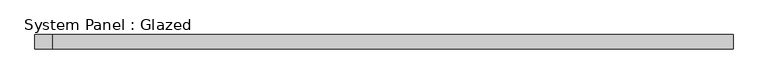
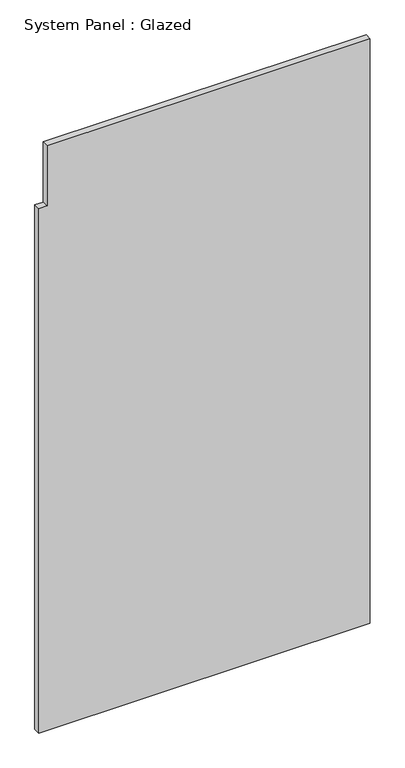
"""IFC4 building model written with IfcOpenShell, lengths in millimetres: plate geometry, System Panel : Glazed."""

from ifc_helpers import new_model, si_unit, frame, origin, place, context, project, spatial, polyline, outline, extrude, source, transform, mapped, element, save


def system_panel_glazed_ae0ed77e(model_context):
    return source(origin(), model_context, "Body", "SweptSolid", [
        extrude(outline(polyline([(0.0, -628.65), (0.0, 628.65), (2101.85, 628.65), (2343.15, 628.65), (2343.15, -596.9), (2101.85, -596.9), (2101.85, -628.65), (0.0, -628.65)])), frame((0.0, -44.45, 0.0), z_axis=(0.0, 1.0, 0.0), x_axis=(0.0, 0.0, 1.0)), (0.0, 0.0, 1.0), 25.4),
    ])


if __name__ == "__main__":
    model = new_model("IFC4")
    model_context = context("Model", 3, world=origin())
    ifc_project = project(units=[si_unit("LENGTHUNIT", "METRE", prefix="MILLI")], contexts=[model_context])
    site = spatial("IfcSite", under=ifc_project)
    building = spatial("IfcBuilding", under=site)
    placement = place(None, origin())
    system_panel_glazed_shape = system_panel_glazed_ae0ed77e(model_context)
    element("IfcPlate", 1, ObjectType="System Panel : Glazed", at=placement, inside=building, context=model_context, shape_type="MappedRepresentation", body=[
        mapped(system_panel_glazed_shape, transform((0.0, 0.0, 0.0), x_axis=(1.0, 0.0, 0.0), y_axis=(0.0, 1.0, 0.0), z_axis=(0.0, 0.0, 1.0))),
    ])
    save(model, "model.ifc")

# Revit data of these elements
# Element 1 (IfcPlate, "System Panel : Glazed")
#   Materials on its faces: "Glass"
# Materials
#   "Glass": class "Glass", colour RGB 0 128 192, transparency 0.75, Cost = 0
